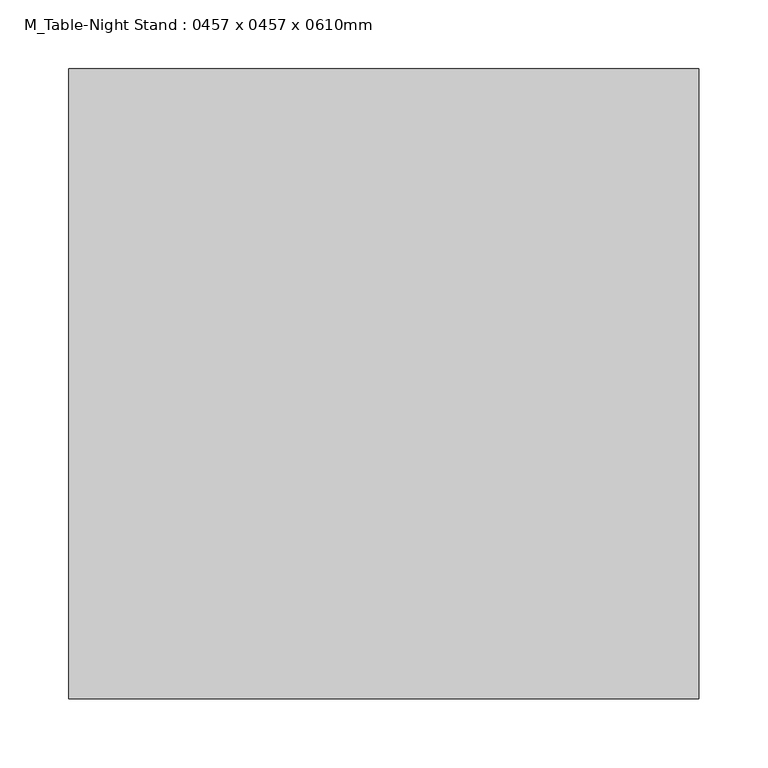
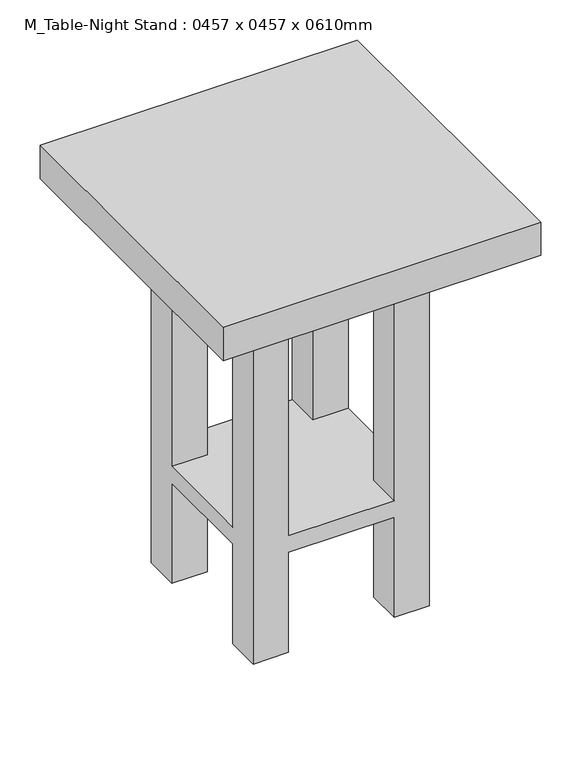
"""IFC4 building model written with IfcOpenShell, lengths in millimetres: furniture geometry, M_Table-Night Stand : 0457 x 0457 x 0610mm."""

import ifcopenshell
import ifcopenshell.guid

model = None  # the IFC model being written
_history = None  # IfcOwnerHistory: only IFC2X3 demands one
_inside = {}  # id of a spatial element -> (the spatial element, [elements in it])
_under = {}  # id of a project, library or spatial element -> (it, [spatial elements below it])
_declared = {}  # id of a project -> (the project, [libraries it declares])
_typed = {}  # id of a type object -> (the type object, [elements of that type])
_made_of = {}  # id of a material, layer set ... -> (it, [elements and type objects made of it])


def new_model(schema):
    """Start an empty IFC model of exactly this schema.

    Asked for "IFC4X3", IfcOpenShell would pick the latest addendum, in which some entities
    have other attributes; the version numbers below select the first issue.
    IFC2X3 requires an IfcOwnerHistory on every rooted entity: one is made here for all.
    """
    global model, _history
    if schema == "IFC4X3":
        model = ifcopenshell.file(schema_version=(4, 3, 0, 0))
    else:
        model = ifcopenshell.file(schema=schema)
    _inside.clear()
    _under.clear()
    _declared.clear()
    _typed.clear()
    _made_of.clear()
    _history = None
    if model.schema == "IFC2X3":
        org = make("IfcOrganization", Name="unknown")
        user = make(
            "IfcPersonAndOrganization",
            ThePerson=make("IfcPerson", FamilyName="unknown"),
            TheOrganization=org,
        )
        app = make(
            "IfcApplication",
            ApplicationDeveloper=org,
            Version="unknown",
            ApplicationFullName="unknown",
            ApplicationIdentifier="unknown",
        )
        _history = make(
            "IfcOwnerHistory",
            OwningUser=user,
            OwningApplication=app,
            ChangeAction="ADDED",
            CreationDate=0,
        )
    return model


def make(cls, **values):
    """One entity of the class cls with the attributes given. An attribute that is None is left unset."""
    return model.create_entity(
        cls, **{name: value for name, value in values.items() if value is not None}
    )


def rooted(cls, **values):
    """An entity with a GlobalId (a new one), such as an element, a storey or a relation."""
    return make(cls, GlobalId=ifcopenshell.guid.new(), OwnerHistory=_history, **values)


def si_unit(unit_type, name, prefix=None):
    """IfcSIUnit, for example si_unit("LENGTHUNIT", "METRE", prefix="MILLI")."""
    return make("IfcSIUnit", UnitType=unit_type, Prefix=prefix, Name=name)


def assignment(units):
    """IfcUnitAssignment: the units of a project."""
    return None if units is None else make("IfcUnitAssignment", Units=units)


def point(xyz):
    """IfcCartesianPoint."""
    return None if xyz is None else make("IfcCartesianPoint", Coordinates=xyz)


def direction(xyz):
    """IfcDirection."""
    return None if xyz is None else make("IfcDirection", DirectionRatios=xyz)


def frame(location, z_axis=None, x_axis=None):
    """IfcAxis2Placement3D, a coordinate frame: its origin and axes. An axis left out is left unset."""
    return make(
        "IfcAxis2Placement3D",
        Location=point(location),
        Axis=direction(z_axis),
        RefDirection=direction(x_axis),
    )


def origin():
    """The frame at (0, 0, 0) with its axes left unset."""
    return frame((0.0, 0.0, 0.0))


def place(relative_to, where):
    """IfcLocalPlacement: puts the frame where relative to a parent placement (None: the world)."""
    return make(
        "IfcLocalPlacement", PlacementRelTo=relative_to, RelativePlacement=where
    )


def context(
    kind, dimensions, precision=None, world=None, true_north=None, identifier=None
):
    """IfcGeometricRepresentationContext, for example the 3D "Model" context."""
    return make(
        "IfcGeometricRepresentationContext",
        ContextIdentifier=identifier,
        ContextType=kind,
        CoordinateSpaceDimension=dimensions,
        Precision=precision,
        WorldCoordinateSystem=world,
        TrueNorth=true_north,
    )


def project(units=None, contexts=None):
    """IfcProject with its units and contexts."""
    return rooted(
        "IfcProject",
        Name="project",
        RepresentationContexts=contexts,
        UnitsInContext=assignment(units),
    )


def spatial(cls, under=None, at=None, **own):
    """A site, building, storey or space (cls), placed at a placement, below another one or the project."""
    s = rooted(cls, ObjectPlacement=at, **own)
    if under is not None:
        _under.setdefault(under.id(), (under, []))[1].append(s)
    return s


def polyline(points):
    """IfcPolyline through the points."""
    return make("IfcPolyline", Points=[point(p) for p in points])


def outline(outer, holes=None, kind="AREA"):
    """IfcArbitraryClosedProfileDef: a profile drawn as a closed curve; with holes, ...WithVoids."""
    if holes is None:
        return make("IfcArbitraryClosedProfileDef", ProfileType=kind, OuterCurve=outer)
    return make(
        "IfcArbitraryProfileDefWithVoids",
        ProfileType=kind,
        OuterCurve=outer,
        InnerCurves=holes,
    )


def extrude(swept, where, along, depth):
    """IfcExtrudedAreaSolid: the profile swept, set in the frame where, extruded along a direction by depth."""
    return make(
        "IfcExtrudedAreaSolid",
        SweptArea=swept,
        Position=where,
        ExtrudedDirection=direction(along),
        Depth=depth,
    )


def faces_of(points, faces, orient=None, outer=None):
    """IfcFace entities. A face is a list of loops; a loop is a list of indices into points, from 0.

    orient and outer hold one flag for each loop. By default every Orientation is true, the
    first loop of a face is its IfcFaceOuterBound and the others are IfcFaceBound.
    """
    made = []
    for i, loops in enumerate(faces):
        bounds = []
        for j, loop in enumerate(loops):
            is_outer = j == 0 if outer is None else outer[i][j]
            bounds.append(
                make(
                    "IfcFaceOuterBound" if is_outer else "IfcFaceBound",
                    Bound=make("IfcPolyLoop", Polygon=[points[k] for k in loop]),
                    Orientation=True if orient is None else orient[i][j],
                )
            )
        made.append(make("IfcFace", Bounds=bounds))
    return made


def faceted_brep(points, faces, orient=None, outer=None, voids=None):
    """IfcFacetedBrep: a solid bounded by flat faces; with voids (closed shells), ...WithVoids."""
    shared = [point(p) for p in points]
    hull = make("IfcClosedShell", CfsFaces=faces_of(shared, faces, orient, outer))
    if voids is None:
        return make("IfcFacetedBrep", Outer=hull)
    return make(
        "IfcFacetedBrepWithVoids",
        Outer=hull,
        Voids=[
            make(cls, CfsFaces=faces_of(shared, fs, o, b)) for cls, fs, o, b in voids
        ],
    )


def shape(context_of_items, identifier, shape_type, items):
    """IfcShapeRepresentation: the items that make up one representation, for example the "Body"."""
    return make(
        "IfcShapeRepresentation",
        ContextOfItems=context_of_items,
        RepresentationIdentifier=identifier,
        RepresentationType=shape_type,
        Items=items,
    )


def source(mapping_origin, context_of_items, identifier, shape_type, items):
    """IfcRepresentationMap: a shape defined once, which mapped items show again and again."""
    return make(
        "IfcRepresentationMap",
        MappingOrigin=mapping_origin,
        MappedRepresentation=shape(context_of_items, identifier, shape_type, items),
    )


def transform(
    local_origin,
    x_axis=None,
    y_axis=None,
    z_axis=None,
    scale=None,
    scale2=None,
    scale3=None,
    uniform=True,
):
    """IfcCartesianTransformationOperator3D, or its non-uniform kind. x_axis, y_axis, z_axis: its Axis1, 2, 3."""
    if uniform:
        return make(
            "IfcCartesianTransformationOperator3D",
            Axis1=direction(x_axis),
            Axis2=direction(y_axis),
            LocalOrigin=point(local_origin),
            Scale=scale,
            Axis3=direction(z_axis),
        )
    return make(
        "IfcCartesianTransformationOperator3DnonUniform",
        Axis1=direction(x_axis),
        Axis2=direction(y_axis),
        LocalOrigin=point(local_origin),
        Scale=scale,
        Axis3=direction(z_axis),
        Scale2=scale2,
        Scale3=scale3,
    )


def mapped(mapping_source, mapping_target):
    """IfcMappedItem: shows the shape of a source again, moved by a transform."""
    return make(
        "IfcMappedItem", MappingSource=mapping_source, MappingTarget=mapping_target
    )


def made_of(thing, what):
    """Note that an element or type object is made of a material, layer set ...; save() writes the relation."""
    if what is not None:
        _made_of.setdefault(what.id(), (what, []))[1].append(thing)
    return thing


def element(
    cls,
    number,
    at=None,
    inside=None,
    cuts=None,
    type_object=None,
    material=None,
    context=None,
    identifier="Body",
    shape_type=None,
    held_by="IfcProductDefinitionShape",
    body=None,
    shapes=None,
    **own,
):
    """One element of the class cls, such as IfcWall. Its Tag is "e" and its number.

    at: its placement. inside: the storey or other place that contains it. cuts: it is an
    opening in that element (IfcRelVoidsElement). A single representation is given by context,
    identifier, shape_type and body (its items); several are given by shapes. held_by: the class
    of the entity that holds the representations. save() writes the other relations.
    """
    e = rooted(cls, Tag="e%d" % number, ObjectPlacement=at, **own)
    if body is not None:
        shapes = [shape(context, identifier, shape_type, body)]
    if shapes is not None:
        e.Representation = make(held_by, Representations=shapes)
    if inside is not None:
        _inside.setdefault(inside.id(), (inside, []))[1].append(e)
    if cuts is not None:
        rooted(
            "IfcRelVoidsElement", RelatingBuildingElement=cuts, RelatedOpeningElement=e
        )
    if type_object is not None:
        _typed.setdefault(type_object.id(), (type_object, []))[1].append(e)
    return made_of(e, material)


def aggregate(whole, parts):
    """IfcRelAggregates: a whole, such as a stair, and the parts it consists of."""
    return rooted("IfcRelAggregates", RelatingObject=whole, RelatedObjects=parts)


def save(model, path):
    """Write the relations noted so far, then the file.

    IfcRelAggregates (storeys below a building ...), IfcRelContainedInSpatialStructure (elements
    in a storey), IfcRelDefinesByType, IfcRelAssociatesMaterial and IfcRelDeclares: one each for
    every whole, place, type object, material and project.
    """
    for whole, parts in _under.values():
        aggregate(whole, parts)
    for where, things in _inside.values():
        rooted(
            "IfcRelContainedInSpatialStructure",
            RelatedElements=things,
            RelatingStructure=where,
        )
    for kind, things in _typed.values():
        rooted("IfcRelDefinesByType", RelatedObjects=things, RelatingType=kind)
    for what, things in _made_of.values():
        rooted("IfcRelAssociatesMaterial", RelatedObjects=things, RelatingMaterial=what)
    for by, libraries in _declared.values():
        rooted("IfcRelDeclares", RelatingContext=by, RelatedDefinitions=libraries)
    model.write(path)


def m_table_night_stand_0457_x_0457_x_0610mm_e3011d0a(model_context):
    return source(origin(), model_context, "Body", "SolidModel", [
        faceted_brep([(156.1336303, 355.4, 559.2), (105.3336303, 355.4, 559.2), (105.3336303, 304.6, 559.2), (156.1336303, 304.6, 559.2), (156.1336303, 152.4, 559.2), (105.3336303, 152.4, 559.2), (105.3336303, 101.6, 559.2), (156.1336303, 101.6, 559.2), (359.1336303, 355.4, 559.2), (308.3336303, 355.4, 559.2), (308.3336303, 304.6, 559.2), (359.1336303, 304.6, 559.2), (359.1336303, 152.4, 559.2), (308.3336303, 152.4, 559.2), (308.3336303, 101.6, 559.2), (359.1336303, 101.6, 559.2), (156.1336303, 355.4, 0.0), (156.1336303, 304.6, 0.0), (105.3336303, 304.6, 0.0), (105.3336303, 355.4, 0.0), (156.1336303, 152.4, 0.0), (156.1336303, 101.6, 0.0), (105.3336303, 101.6, 0.0), (105.3336303, 152.4, 0.0), (359.1336303, 355.4, 0.0), (359.1336303, 304.6, 0.0), (308.3336303, 304.6, 0.0), (308.3336303, 355.4, 0.0), (359.1336303, 152.4, 0.0), (359.1336303, 101.6, 0.0), (308.3336303, 101.6, 0.0), (308.3336303, 152.4, 0.0), (156.1336303, 355.4, 177.8), (308.3336303, 355.4, 177.8), (308.3336303, 355.4, 152.4), (156.1336303, 355.4, 152.4), (105.3336303, 304.6, 152.4), (105.3336303, 152.4, 152.4), (105.3336303, 152.4, 177.8), (105.3336303, 304.6, 177.8), (156.1336303, 304.6, 177.8), (156.1336303, 304.6, 152.4), (156.1336303, 152.4, 177.8), (156.1336303, 152.4, 152.4), (156.1336303, 101.6, 152.4), (308.3336303, 101.6, 152.4), (308.3336303, 101.6, 177.8), (156.1336303, 101.6, 177.8), (308.3336303, 304.6, 177.8), (308.3336303, 304.6, 152.4), (359.1336303, 304.6, 177.8), (359.1336303, 304.6, 152.4), (359.1336303, 152.4, 177.8), (359.1336303, 152.4, 152.4), (308.3336303, 152.4, 177.8), (308.3336303, 152.4, 152.4)], [[[0, 1, 2, 3]], [[4, 5, 6, 7]], [[8, 9, 10, 11]], [[12, 13, 14, 15]], [[16, 17, 18, 19]], [[20, 21, 22, 23]], [[24, 25, 26, 27]], [[28, 29, 30, 31]], [[1, 0, 32, 33, 9, 8, 24, 27, 34, 35, 16, 19]], [[2, 1, 19, 18, 36, 37, 23, 22, 6, 5, 38, 39]], [[3, 2, 39, 40]], [[18, 17, 41, 36]], [[0, 3, 40, 32]], [[17, 16, 35, 41]], [[5, 4, 42, 38]], [[20, 23, 37, 43]], [[7, 6, 22, 21, 44, 45, 30, 29, 15, 14, 46, 47]], [[4, 7, 47, 42]], [[21, 20, 43, 44]], [[10, 9, 33, 48]], [[27, 26, 49, 34]], [[11, 10, 48, 50]], [[26, 25, 51, 49]], [[8, 11, 50, 52, 12, 15, 29, 28, 53, 51, 25, 24]], [[13, 12, 52, 54]], [[28, 31, 55, 53]], [[14, 13, 54, 46]], [[31, 30, 45, 55]], [[39, 38, 42, 47, 46, 54, 52, 50, 48, 33, 32, 40]], [[35, 34, 49, 51, 53, 55, 45, 44, 43, 37, 36, 41]]]),
        extrude(outline(polyline([(460.7336303, 0.0), (3.7336303, 0.0), (3.7336303, 457.0), (460.7336303, 457.0), (460.7336303, 0.0)])), frame((0.0, 0.0, 559.2), z_axis=(0.0, 0.0, 1.0), x_axis=(1.0, 0.0, 0.0)), (0.0, 0.0, 1.0), 50.8),
    ])


if __name__ == "__main__":
    model = new_model("IFC4")
    model_context = context("Model", 3, world=origin())
    ifc_project = project(units=[si_unit("LENGTHUNIT", "METRE", prefix="MILLI")], contexts=[model_context])
    site = spatial("IfcSite", under=ifc_project)
    building = spatial("IfcBuilding", under=site)
    placement = place(None, origin())
    m_table_night_stand_0457_x_0457_x_0610mm_shape = m_table_night_stand_0457_x_0457_x_0610mm_e3011d0a(model_context)
    element("IfcFurniture", 1, ObjectType="M_Table-Night Stand : 0457 x 0457 x 0610mm", at=placement, inside=building, context=model_context, shape_type="MappedRepresentation", body=[
        mapped(m_table_night_stand_0457_x_0457_x_0610mm_shape, transform((0.0, 0.0, 0.0), x_axis=(1.0, 0.0, 0.0), y_axis=(0.0, 1.0, 0.0), z_axis=(0.0, 0.0, 1.0))),
    ])
    save(model, "model.ifc")

# Revit data of these elements
# Type "M_Table-Night Stand : 0457 x 0457 x 0610mm"
#   Depth = 0.457 m
#   Height = 0.61 m
#   Width = 0.457 m
#   Base Material = Birch
#   Top Material = Laminate, Ivory, Matte
# Element 1 (IfcFurniture, "M_Table-Night Stand : 0457 x 0457 x 0610mm")
#   Materials on its faces: "Birch", "Laminate, Ivory, Matte"
# Materials
#   "Birch": class "Wood", colour RGB 224 178 126, transparency 0, Description = "Betula Alleghaniensis", Cost = 0
#   "Laminate, Ivory, Matte": class "Plastic", colour RGB 247 247 239, transparency 0, Description = "Plastic Laminate - Ivory, Matte", Cost = 0
